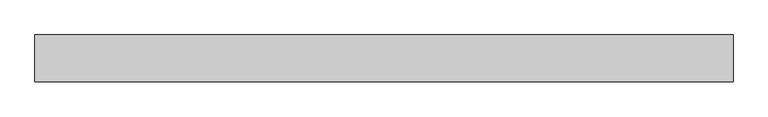
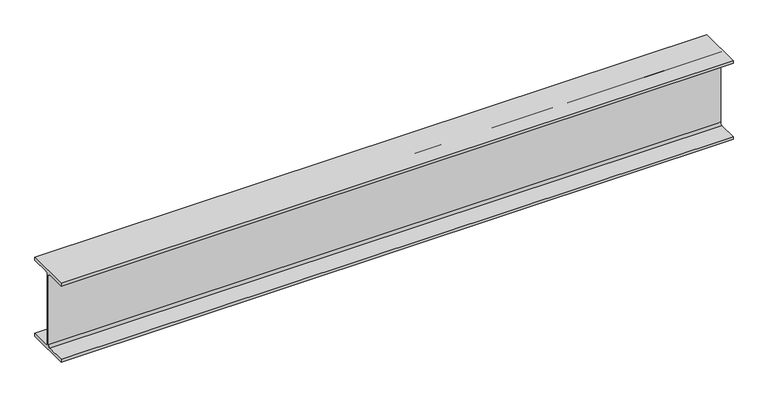
"""IFC4 building model written with IfcOpenShell, lengths in millimetres: beam geometry, Old_Steel Beam_H-KSD3502 : H_SB_ASB_H-194×150x6x9."""

from ifc_helpers import new_model, si_unit, point, frame, frame_2d, origin, place, context, project, spatial, polyline, circle_curve, trimmed, segment, composite_curve, outline, extrude, source, transform, mapped, element, save


def beam_e3c91eea(model_context):
    return source(origin(), model_context, "Body", "SweptSolid", [
        extrude(outline(composite_curve([segment(polyline([(-82.5, -141.5), (-11.9, -141.5)]), True, "CONTINUOUS"), segment(trimmed(circle_curve(frame_2d((-11.9, -132.6)), 8.9), [point((-11.9, -141.5))], [point((-3.0, -132.6))], True, "CARTESIAN"), True, "CONTINUOUS"), segment(polyline([(-3.0, -132.6), (-3.0, 132.6)]), True, "CONTINUOUS"), segment(trimmed(circle_curve(frame_2d((-11.9, 132.6)), 8.9), [point((-3.0, 132.6))], [point((-11.9, 141.5))], True, "CARTESIAN"), True, "CONTINUOUS"), segment(polyline([(-11.9, 141.5), (-82.5, 141.5), (-82.5, 151.7), (82.5, 151.7), (82.5, 141.5), (11.9, 141.5)]), True, "CONTINUOUS"), segment(trimmed(circle_curve(frame_2d((11.9, 132.6)), 8.9), [point((11.9, 141.5))], [point((3.0, 132.6))], True, "CARTESIAN"), True, "CONTINUOUS"), segment(polyline([(3.0, 132.6), (3.0, -132.6)]), True, "CONTINUOUS"), segment(trimmed(circle_curve(frame_2d((11.9, -132.6)), 8.9), [point((3.0, -132.6))], [point((11.9, -141.5))], True, "CARTESIAN"), True, "CONTINUOUS"), segment(polyline([(11.9, -141.5), (82.5, -141.5), (82.5, -151.7), (-82.5, -151.7), (-82.5, -141.5)]), True, "CONTINUOUS")], self_intersect=False)), frame((-1200.0, 0.0, 0.0), z_axis=(1.0, 0.0, 0.0), x_axis=(0.0, 1.0, 0.0)), (0.0, 0.0, 1.0), 2453.1701073),
    ])


if __name__ == "__main__":
    model = new_model("IFC4")
    model_context = context("Model", 3, world=origin())
    ifc_project = project(units=[si_unit("LENGTHUNIT", "METRE", prefix="MILLI")], contexts=[model_context])
    site = spatial("IfcSite", under=ifc_project)
    building = spatial("IfcBuilding", under=site)
    placement = place(None, origin())
    beam_shape = beam_e3c91eea(model_context)
    element("IfcBeam", 1, ObjectType="Old_Steel Beam_H-KSD3502 : H_SB_ASB_H-194×150x6x9", at=placement, inside=building, context=model_context, shape_type="MappedRepresentation", body=[
        mapped(beam_shape, transform((0.0, 0.0, 0.0), x_axis=(1.0, 0.0, 0.0), y_axis=(0.0, 1.0, 0.0), z_axis=(0.0, 0.0, 1.0))),
    ])
    save(model, "model.ifc")

# Revit data of these elements
# Type "Old_Steel Beam_H-KSD3502 : H_SB_ASB_H-194×150x6x9"
#   Width = 15.0 cm
#   Web Thickness = 0.6 cm
#   Web Fillet = 1.3 cm
#   Warping Constant = 43316.0 cm⁶
#   Torsional Moment of Inertia = 8.622 cm⁴
#   Torsional Modulus = 1.0 cm³
#   Section Area = 39.01 cm²
#   Plastic Modulus weak axis = 104.0 cm³
#   Plastic Modulus strong axis = 309.0 cm³
#   Perimeter = 0.95 m²/m
#   Nominal Weight = 30.60 kgf/m
#   Moment of Inertia weak axis = 507.00 cm⁴
#   Moment of Inertia strong axis = 2690.00 cm⁴
#   Height = 19.4 cm
#   Flange Thickness = 0.9 cm
#   Elastic Modulus weak axis = 67.6 cm³
#   Elastic Modulus strong axis = 277.0 cm³
#   Centroid Vertical = 9.7 cm
#   Centroid Horizontal = 7.5 cm
#   Length [instance default] = 1.5240 m
#   Structural Material [instance default] = Steel, 45-345
#   Assembly Code = ""
# Element 1 (IfcBeam, "Old_Steel Beam_H-KSD3502 : H_SB_ASB_H-194×150x6x9")
#   Structural Material = none
# Materials
#   "Steel, 45-345": class "Metal", colour RGB 189 187 185, transparency 0, Description = "Steel 345 MPa", Cost = 0
